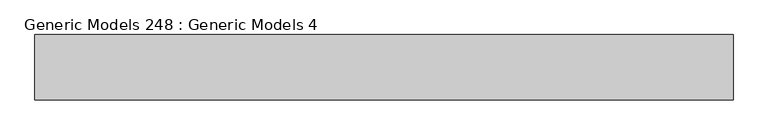
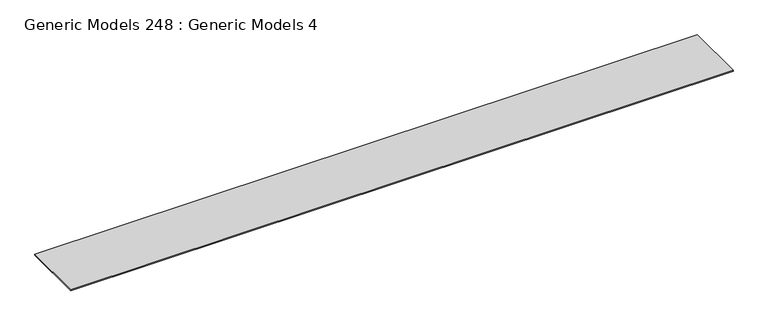
"""IFC4 building model written with IfcOpenShell, lengths in millimetres: proxy geometry, Generic Models 248 : Generic Models 4."""

from ifc_helpers import new_model, si_unit, frame, origin, place, context, project, spatial, polyline, outline, extrude, source, transform, mapped, element, save


def generic_models_248_generic_models_4_1a11a9d1(model_context):
    return source(origin(), model_context, "Body", "SweptSolid", [
        extrude(outline(polyline([(1898.6191326, 11810.9577434), (1898.6191326, 10666.379895), (-10344.1808674, 10666.379895), (-10344.1808674, 11810.9577434), (1898.6191326, 11810.9577434)])), frame((0.0, 0.0, 126364.746), z_axis=(0.0, 0.0, 1.0), x_axis=(1.0, 0.0, 0.0)), (0.0, 0.0, 1.0), 19.05),
    ])


if __name__ == "__main__":
    model = new_model("IFC4")
    model_context = context("Model", 3, world=origin())
    ifc_project = project(units=[si_unit("LENGTHUNIT", "METRE", prefix="MILLI")], contexts=[model_context])
    site = spatial("IfcSite", under=ifc_project)
    building = spatial("IfcBuilding", under=site)
    placement = place(None, origin())
    generic_models_248_generic_models_4_shape = generic_models_248_generic_models_4_1a11a9d1(model_context)
    element("IfcBuildingElementProxy", 1, Name="Generic Models 248 : Generic Models 4", ObjectType="Generic Models 248 : Generic Models 4", at=placement, inside=building, context=model_context, shape_type="MappedRepresentation", body=[
        mapped(generic_models_248_generic_models_4_shape, transform((0.0, 0.0, 0.0), x_axis=(1.0, 0.0, 0.0), y_axis=(0.0, 1.0, 0.0), z_axis=(0.0, 0.0, 1.0))),
    ])
    save(model, "model.ifc")

# Revit data of these elements
# Element 1 (IfcBuildingElementProxy, "Generic Models 248 : Generic Models 4")
#   Materials on its faces: "FIRE RETARDANT TREATED WOOD SOFFIT"
# Materials
#   "FIRE RETARDANT TREATED WOOD SOFFIT": class "Generic", colour RGB 177 130 114, transparency 0, Cost = 0
